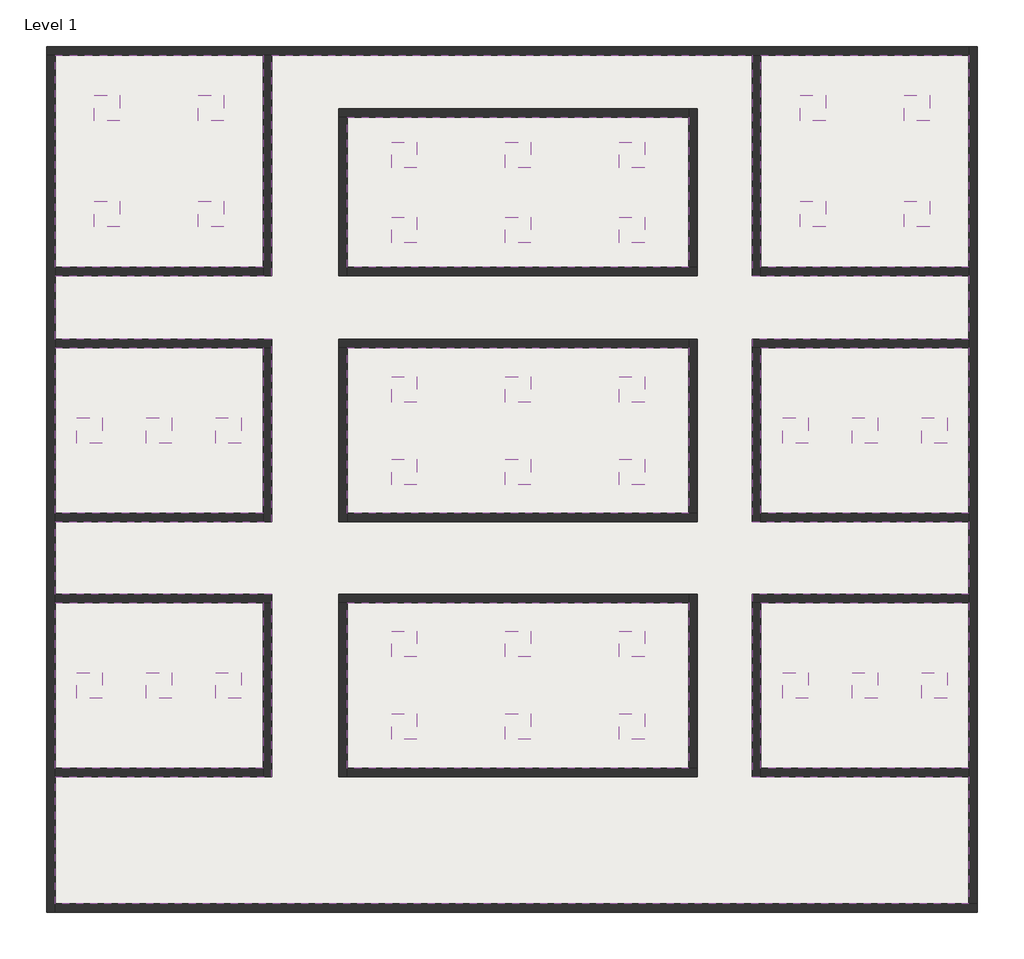
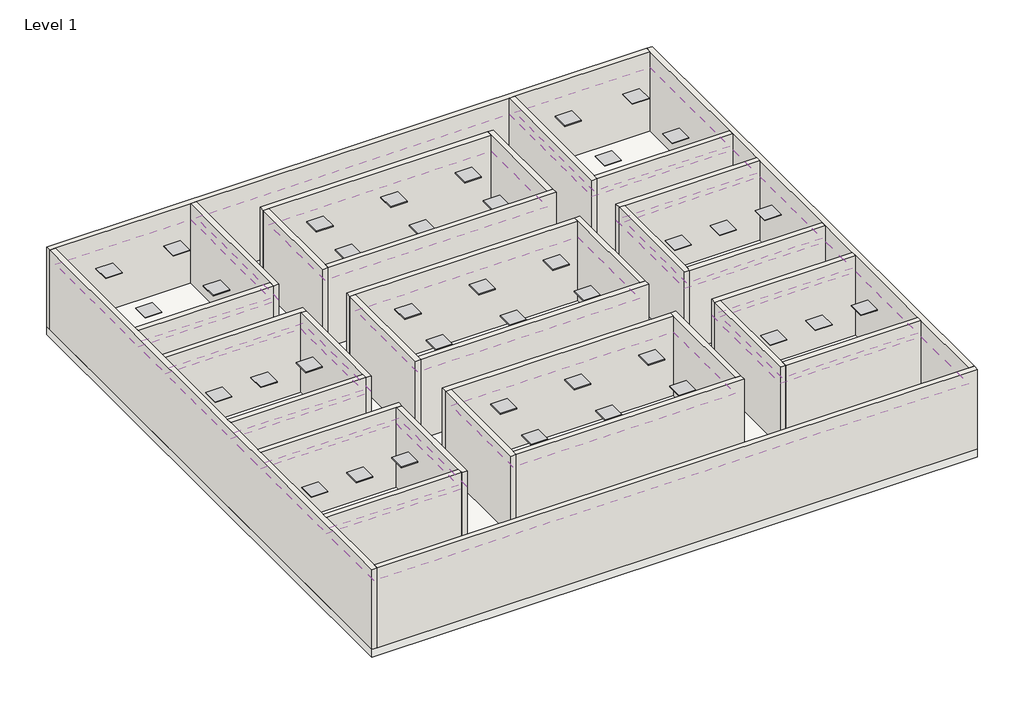
# One storey: 38 light fixtures, 32 walls, 11 coverings, 1 slab.
"""IFC4 building model written with IfcOpenShell, lengths in millimetres."""

import ifcopenshell
import ifcopenshell.guid

model = None  # the IFC model being written
_history = None  # IfcOwnerHistory: only IFC2X3 demands one
_inside = {}  # id of a spatial element -> (the spatial element, [elements in it])
_under = {}  # id of a project, library or spatial element -> (it, [spatial elements below it])
_declared = {}  # id of a project -> (the project, [libraries it declares])
_typed = {}  # id of a type object -> (the type object, [elements of that type])
_made_of = {}  # id of a material, layer set ... -> (it, [elements and type objects made of it])


def new_model(schema):
    """Start an empty IFC model of exactly this schema.

    Asked for "IFC4X3", IfcOpenShell would pick the latest addendum, in which some entities
    have other attributes; the version numbers below select the first issue.
    IFC2X3 requires an IfcOwnerHistory on every rooted entity: one is made here for all.
    """
    global model, _history
    if schema == "IFC4X3":
        model = ifcopenshell.file(schema_version=(4, 3, 0, 0))
    else:
        model = ifcopenshell.file(schema=schema)
    _inside.clear()
    _under.clear()
    _declared.clear()
    _typed.clear()
    _made_of.clear()
    _history = None
    if model.schema == "IFC2X3":
        org = make("IfcOrganization", Name="unknown")
        user = make(
            "IfcPersonAndOrganization",
            ThePerson=make("IfcPerson", FamilyName="unknown"),
            TheOrganization=org,
        )
        app = make(
            "IfcApplication",
            ApplicationDeveloper=org,
            Version="unknown",
            ApplicationFullName="unknown",
            ApplicationIdentifier="unknown",
        )
        _history = make(
            "IfcOwnerHistory",
            OwningUser=user,
            OwningApplication=app,
            ChangeAction="ADDED",
            CreationDate=0,
        )
    return model


def make(cls, **values):
    """One entity of the class cls with the attributes given. An attribute that is None is left unset."""
    return model.create_entity(
        cls, **{name: value for name, value in values.items() if value is not None}
    )


def rooted(cls, **values):
    """An entity with a GlobalId (a new one), such as an element, a storey or a relation."""
    return make(cls, GlobalId=ifcopenshell.guid.new(), OwnerHistory=_history, **values)


def si_unit(unit_type, name, prefix=None):
    """IfcSIUnit, for example si_unit("LENGTHUNIT", "METRE", prefix="MILLI")."""
    return make("IfcSIUnit", UnitType=unit_type, Prefix=prefix, Name=name)


def assignment(units):
    """IfcUnitAssignment: the units of a project."""
    return None if units is None else make("IfcUnitAssignment", Units=units)


def point(xyz):
    """IfcCartesianPoint."""
    return None if xyz is None else make("IfcCartesianPoint", Coordinates=xyz)


def direction(xyz):
    """IfcDirection."""
    return None if xyz is None else make("IfcDirection", DirectionRatios=xyz)


def frame(location, z_axis=None, x_axis=None):
    """IfcAxis2Placement3D, a coordinate frame: its origin and axes. An axis left out is left unset."""
    return make(
        "IfcAxis2Placement3D",
        Location=point(location),
        Axis=direction(z_axis),
        RefDirection=direction(x_axis),
    )


def origin():
    """The frame at (0, 0, 0) with its axes left unset."""
    return frame((0.0, 0.0, 0.0))


def origin_with_axes():
    """The frame at (0, 0, 0) with the z axis (0, 0, 1) and the x axis (1, 0, 0) written out."""
    return frame((0.0, 0.0, 0.0), z_axis=(0.0, 0.0, 1.0), x_axis=(1.0, 0.0, 0.0))


def place(relative_to, where):
    """IfcLocalPlacement: puts the frame where relative to a parent placement (None: the world)."""
    return make(
        "IfcLocalPlacement", PlacementRelTo=relative_to, RelativePlacement=where
    )


def context(
    kind, dimensions, precision=None, world=None, true_north=None, identifier=None
):
    """IfcGeometricRepresentationContext, for example the 3D "Model" context."""
    return make(
        "IfcGeometricRepresentationContext",
        ContextIdentifier=identifier,
        ContextType=kind,
        CoordinateSpaceDimension=dimensions,
        Precision=precision,
        WorldCoordinateSystem=world,
        TrueNorth=true_north,
    )


def project(units=None, contexts=None):
    """IfcProject with its units and contexts."""
    return rooted(
        "IfcProject",
        Name="project",
        RepresentationContexts=contexts,
        UnitsInContext=assignment(units),
    )


def spatial(cls, under=None, at=None, **own):
    """A site, building, storey or space (cls), placed at a placement, below another one or the project."""
    s = rooted(cls, ObjectPlacement=at, **own)
    if under is not None:
        _under.setdefault(under.id(), (under, []))[1].append(s)
    return s


def polyline(points):
    """IfcPolyline through the points."""
    return make("IfcPolyline", Points=[point(p) for p in points])


def outline(outer, holes=None, kind="AREA"):
    """IfcArbitraryClosedProfileDef: a profile drawn as a closed curve; with holes, ...WithVoids."""
    if holes is None:
        return make("IfcArbitraryClosedProfileDef", ProfileType=kind, OuterCurve=outer)
    return make(
        "IfcArbitraryProfileDefWithVoids",
        ProfileType=kind,
        OuterCurve=outer,
        InnerCurves=holes,
    )


def extrude(swept, where, along, depth):
    """IfcExtrudedAreaSolid: the profile swept, set in the frame where, extruded along a direction by depth."""
    return make(
        "IfcExtrudedAreaSolid",
        SweptArea=swept,
        Position=where,
        ExtrudedDirection=direction(along),
        Depth=depth,
    )


def faces_of(points, faces, orient=None, outer=None):
    """IfcFace entities. A face is a list of loops; a loop is a list of indices into points, from 0.

    orient and outer hold one flag for each loop. By default every Orientation is true, the
    first loop of a face is its IfcFaceOuterBound and the others are IfcFaceBound.
    """
    made = []
    for i, loops in enumerate(faces):
        bounds = []
        for j, loop in enumerate(loops):
            is_outer = j == 0 if outer is None else outer[i][j]
            bounds.append(
                make(
                    "IfcFaceOuterBound" if is_outer else "IfcFaceBound",
                    Bound=make("IfcPolyLoop", Polygon=[points[k] for k in loop]),
                    Orientation=True if orient is None else orient[i][j],
                )
            )
        made.append(make("IfcFace", Bounds=bounds))
    return made


def faceted_brep(points, faces, orient=None, outer=None, voids=None):
    """IfcFacetedBrep: a solid bounded by flat faces; with voids (closed shells), ...WithVoids."""
    shared = [point(p) for p in points]
    hull = make("IfcClosedShell", CfsFaces=faces_of(shared, faces, orient, outer))
    if voids is None:
        return make("IfcFacetedBrep", Outer=hull)
    return make(
        "IfcFacetedBrepWithVoids",
        Outer=hull,
        Voids=[
            make(cls, CfsFaces=faces_of(shared, fs, o, b)) for cls, fs, o, b in voids
        ],
    )


def shape(context_of_items, identifier, shape_type, items):
    """IfcShapeRepresentation: the items that make up one representation, for example the "Body"."""
    return make(
        "IfcShapeRepresentation",
        ContextOfItems=context_of_items,
        RepresentationIdentifier=identifier,
        RepresentationType=shape_type,
        Items=items,
    )


def source(mapping_origin, context_of_items, identifier, shape_type, items):
    """IfcRepresentationMap: a shape defined once, which mapped items show again and again."""
    return make(
        "IfcRepresentationMap",
        MappingOrigin=mapping_origin,
        MappedRepresentation=shape(context_of_items, identifier, shape_type, items),
    )


def transform(
    local_origin,
    x_axis=None,
    y_axis=None,
    z_axis=None,
    scale=None,
    scale2=None,
    scale3=None,
    uniform=True,
):
    """IfcCartesianTransformationOperator3D, or its non-uniform kind. x_axis, y_axis, z_axis: its Axis1, 2, 3."""
    if uniform:
        return make(
            "IfcCartesianTransformationOperator3D",
            Axis1=direction(x_axis),
            Axis2=direction(y_axis),
            LocalOrigin=point(local_origin),
            Scale=scale,
            Axis3=direction(z_axis),
        )
    return make(
        "IfcCartesianTransformationOperator3DnonUniform",
        Axis1=direction(x_axis),
        Axis2=direction(y_axis),
        LocalOrigin=point(local_origin),
        Scale=scale,
        Axis3=direction(z_axis),
        Scale2=scale2,
        Scale3=scale3,
    )


def mapped(mapping_source, mapping_target):
    """IfcMappedItem: shows the shape of a source again, moved by a transform."""
    return make(
        "IfcMappedItem", MappingSource=mapping_source, MappingTarget=mapping_target
    )


def made_of(thing, what):
    """Note that an element or type object is made of a material, layer set ...; save() writes the relation."""
    if what is not None:
        _made_of.setdefault(what.id(), (what, []))[1].append(thing)
    return thing


def element(
    cls,
    number,
    at=None,
    inside=None,
    cuts=None,
    type_object=None,
    material=None,
    context=None,
    identifier="Body",
    shape_type=None,
    held_by="IfcProductDefinitionShape",
    body=None,
    shapes=None,
    **own,
):
    """One element of the class cls, such as IfcWall. Its Tag is "e" and its number.

    at: its placement. inside: the storey or other place that contains it. cuts: it is an
    opening in that element (IfcRelVoidsElement). A single representation is given by context,
    identifier, shape_type and body (its items); several are given by shapes. held_by: the class
    of the entity that holds the representations. save() writes the other relations.
    """
    e = rooted(cls, Tag="e%d" % number, ObjectPlacement=at, **own)
    if body is not None:
        shapes = [shape(context, identifier, shape_type, body)]
    if shapes is not None:
        e.Representation = make(held_by, Representations=shapes)
    if inside is not None:
        _inside.setdefault(inside.id(), (inside, []))[1].append(e)
    if cuts is not None:
        rooted(
            "IfcRelVoidsElement", RelatingBuildingElement=cuts, RelatedOpeningElement=e
        )
    if type_object is not None:
        _typed.setdefault(type_object.id(), (type_object, []))[1].append(e)
    return made_of(e, material)


def aggregate(whole, parts):
    """IfcRelAggregates: a whole, such as a stair, and the parts it consists of."""
    return rooted("IfcRelAggregates", RelatingObject=whole, RelatedObjects=parts)


def save(model, path):
    """Write the relations noted so far, then the file.

    IfcRelAggregates (storeys below a building ...), IfcRelContainedInSpatialStructure (elements
    in a storey), IfcRelDefinesByType, IfcRelAssociatesMaterial and IfcRelDeclares: one each for
    every whole, place, type object, material and project.
    """
    for whole, parts in _under.values():
        aggregate(whole, parts)
    for where, things in _inside.values():
        rooted(
            "IfcRelContainedInSpatialStructure",
            RelatedElements=things,
            RelatingStructure=where,
        )
    for kind, things in _typed.values():
        rooted("IfcRelDefinesByType", RelatedObjects=things, RelatingType=kind)
    for what, things in _made_of.values():
        rooted("IfcRelAssociatesMaterial", RelatedObjects=things, RelatingMaterial=what)
    for by, libraries in _declared.values():
        rooted("IfcRelDeclares", RelatingContext=by, RelatedDefinitions=libraries)
    model.write(path)


def simple_lights_a_61f39cf9(model_context):
    return source(origin(), model_context, "Body", "SweptSolid", [
        extrude(outline(polyline([(300.0, 300.0), (300.0, -300.0), (-300.0, -300.0), (-300.0, 300.0), (300.0, 300.0)])), frame((0.0, 0.0, -30.0), z_axis=(0.0, 0.0, 1.0), x_axis=(1.0, 0.0, 0.0)), (0.0, 0.0, 1.0), 30.0),
    ])


model = new_model("IFC4")

# Units and contexts
model_context = context("Model", 3, world=origin())
ifc_project = project(units=[si_unit("LENGTHUNIT", "METRE", prefix="MILLI")], contexts=[model_context])

# Site, building, storey
site = spatial("IfcSite", under=ifc_project)
building = spatial("IfcBuilding", under=site)
storey = spatial("IfcBuildingStorey", under=building, Name="Level 1", Elevation=0.0)

# Coverings
placement = place(None, origin())
element("IfcCovering", 1, ObjectType="2' x 4' ACT System", at=placement, inside=storey, context=model_context, shape_type="SweptSolid", body=[
    extrude(outline(polyline([(-11709.662063, 12460.3552234), (-6809.662063, 12460.3552234), (-6809.662063, 7460.3552234), (-11709.662063, 7460.3552234), (-11709.662063, 12460.3552234)])), frame((0.0, 0.0, 2438.4), z_axis=(0.0, 0.0, 1.0), x_axis=(1.0, 0.0, 0.0)), (0.0, 0.0, 1.0), 57.15),
])
element("IfcCovering", 2, ObjectType="2' x 4' ACT System", at=placement, inside=storey, context=model_context, shape_type="SweptSolid", body=[
    extrude(outline(polyline([(-6609.662063, 7260.3552234), (-6609.662063, 12460.3552234), (4722.664183, 12460.3552234), (4722.664183, 7260.3552234), (9822.664183, 7260.3552234), (9822.664183, 5760.3552234), (4722.664183, 5760.3552234), (4722.664183, 1460.3552234), (9822.664183, 1460.3552234), (9822.664183, -239.6447766), (4722.664183, -239.6447766), (4722.664183, -4539.6447766), (9822.664183, -4539.6447766), (9822.664183, -7539.6447766), (-11709.662063, -7539.6447766), (-11709.662063, -4539.6447766), (-6609.662063, -4539.6447766), (-6609.662063, -239.6447766), (-11709.662063, -239.6447766), (-11709.662063, 1460.3552234), (-6609.662063, 1460.3552234), (-6609.662063, 5760.3552234), (-11709.662063, 5760.3552234), (-11709.662063, 7260.3552234), (-6609.662063, 7260.3552234)]), holes=[polyline([(3422.664183, 7260.3552234), (3422.664183, 11191.3898121), (-5023.4293583, 11191.3898121), (-5023.4293583, 7260.3552234), (3422.664183, 7260.3552234)]), polyline([(3422.664183, 1460.3552234), (3422.664183, 5760.3552234), (-5023.4293583, 5760.3552234), (-5023.4293583, 1460.3552234), (3422.664183, 1460.3552234)]), polyline([(3422.664183, -4539.6447766), (3422.664183, -239.6447766), (-5023.4293583, -239.6447766), (-5023.4293583, -4539.6447766), (3422.664183, -4539.6447766)])]), frame((0.0, 0.0, 2438.4), z_axis=(0.0, 0.0, 1.0), x_axis=(1.0, 0.0, 0.0)), (0.0, 0.0, 1.0), 57.15),
])
element("IfcCovering", 3, ObjectType="2' x 4' ACT System", at=placement, inside=storey, context=model_context, shape_type="SweptSolid", body=[
    extrude(outline(polyline([(-4823.4293583, 10991.3898121), (3222.664183, 10991.3898121), (3222.664183, 7460.3552234), (-4823.4293583, 7460.3552234), (-4823.4293583, 10991.3898121)])), frame((0.0, 0.0, 2438.4), z_axis=(0.0, 0.0, 1.0), x_axis=(1.0, 0.0, 0.0)), (0.0, 0.0, 1.0), 57.15),
])
element("IfcCovering", 4, ObjectType="2' x 4' ACT System", at=placement, inside=storey, context=model_context, shape_type="SweptSolid", body=[
    extrude(outline(polyline([(4922.664183, 7460.3552234), (4922.664183, 12460.3552234), (9822.664183, 12460.3552234), (9822.664183, 7460.3552234), (4922.664183, 7460.3552234)])), frame((0.0, 0.0, 2438.4), z_axis=(0.0, 0.0, 1.0), x_axis=(1.0, 0.0, 0.0)), (0.0, 0.0, 1.0), 57.15),
])
element("IfcCovering", 5, ObjectType="2' x 4' ACT System", at=placement, inside=storey, context=model_context, shape_type="SweptSolid", body=[
    extrude(outline(polyline([(4922.664183, 5560.3552234), (9822.664183, 5560.3552234), (9822.664183, 1660.3552234), (4922.664183, 1660.3552234), (4922.664183, 5560.3552234)])), frame((0.0, 0.0, 2438.4), z_axis=(0.0, 0.0, 1.0), x_axis=(1.0, 0.0, 0.0)), (0.0, 0.0, 1.0), 57.15),
])
element("IfcCovering", 6, ObjectType="2' x 4' ACT System", at=placement, inside=storey, context=model_context, shape_type="SweptSolid", body=[
    extrude(outline(polyline([(4922.664183, -439.6447766), (9822.664183, -439.6447766), (9822.664183, -4339.6447766), (4922.664183, -4339.6447766), (4922.664183, -439.6447766)])), frame((0.0, 0.0, 2438.4), z_axis=(0.0, 0.0, 1.0), x_axis=(1.0, 0.0, 0.0)), (0.0, 0.0, 1.0), 57.15),
])
element("IfcCovering", 7, ObjectType="2' x 4' ACT System", at=placement, inside=storey, context=model_context, shape_type="SweptSolid", body=[
    extrude(outline(polyline([(-4823.4293583, -439.6447766), (3222.664183, -439.6447766), (3222.664183, -4339.6447766), (-4823.4293583, -4339.6447766), (-4823.4293583, -439.6447766)])), frame((0.0, 0.0, 2438.4), z_axis=(0.0, 0.0, 1.0), x_axis=(1.0, 0.0, 0.0)), (0.0, 0.0, 1.0), 57.15),
])
element("IfcCovering", 8, ObjectType="2' x 4' ACT System", at=placement, inside=storey, context=model_context, shape_type="SweptSolid", body=[
    extrude(outline(polyline([(-11709.662063, -4339.6447766), (-11709.662063, -439.6447766), (-6809.662063, -439.6447766), (-6809.662063, -4339.6447766), (-11709.662063, -4339.6447766)])), frame((0.0, 0.0, 2438.4), z_axis=(0.0, 0.0, 1.0), x_axis=(1.0, 0.0, 0.0)), (0.0, 0.0, 1.0), 57.15),
])
element("IfcCovering", 9, ObjectType="2' x 4' ACT System", at=placement, inside=storey, context=model_context, shape_type="SweptSolid", body=[
    extrude(outline(polyline([(-11709.662063, 1660.3552234), (-11709.662063, 5560.3552234), (-6809.662063, 5560.3552234), (-6809.662063, 1660.3552234), (-11709.662063, 1660.3552234)])), frame((0.0, 0.0, 2438.4), z_axis=(0.0, 0.0, 1.0), x_axis=(1.0, 0.0, 0.0)), (0.0, 0.0, 1.0), 57.15),
])
element("IfcCovering", 10, ObjectType="2' x 4' ACT System", at=placement, inside=storey, context=model_context, shape_type="SweptSolid", body=[
    extrude(outline(polyline([(-4823.4293583, 5560.3552234), (3222.664183, 5560.3552234), (3222.664183, 1660.3552234), (-4823.4293583, 1660.3552234), (-4823.4293583, 5560.3552234)])), frame((0.0, 0.0, 2438.4), z_axis=(0.0, 0.0, 1.0), x_axis=(1.0, 0.0, 0.0)), (0.0, 0.0, 1.0), 57.15),
])
element("IfcCovering", 11, ObjectType="2' x 4' ACT System", at=placement, inside=storey, context=model_context, shape_type="SweptSolid", body=[
    extrude(outline(polyline([(4922.664183, 5560.3552234), (9822.664183, 5560.3552234), (9822.664183, 1660.3552234), (4922.664183, 1660.3552234), (4922.664183, 5560.3552234)])), frame((0.0, 0.0, 2438.4), z_axis=(0.0, 0.0, 1.0), x_axis=(1.0, 0.0, 0.0)), (0.0, 0.0, 1.0), 57.15),
])

# Light fixtures
simple_lights_a_shape = simple_lights_a_61f39cf9(model_context)
element("IfcLightFixture", 12, ObjectType="Simple Lights : A", at=placement, inside=storey, context=model_context, shape_type="MappedRepresentation", body=[
    mapped(simple_lights_a_shape, transform((-10892.9953964, -2389.6447766, 2531.4000022), x_axis=(1.0, 0.0, 0.0), y_axis=(0.0, 1.0, 0.0), z_axis=(0.0, 0.0, 1.0))),
])
element("IfcLightFixture", 13, ObjectType="Simple Lights : A", at=placement, inside=storey, context=model_context, shape_type="MappedRepresentation", body=[
    mapped(simple_lights_a_shape, transform((-9259.662063, -2389.6447766, 2531.4000022), x_axis=(1.0, 0.0, 0.0), y_axis=(0.0, 1.0, 0.0), z_axis=(0.0, 0.0, 1.0))),
])
element("IfcLightFixture", 14, ObjectType="Simple Lights : A", at=placement, inside=storey, context=model_context, shape_type="MappedRepresentation", body=[
    mapped(simple_lights_a_shape, transform((-7626.3287297, -2389.6447766, 2531.4000022), x_axis=(1.0, 0.0, 0.0), y_axis=(0.0, 1.0, 0.0), z_axis=(0.0, 0.0, 1.0))),
])
element("IfcLightFixture", 15, ObjectType="Simple Lights : A", at=placement, inside=storey, context=model_context, shape_type="MappedRepresentation", body=[
    mapped(simple_lights_a_shape, transform((-3482.4137681, -3364.6447766, 2531.4000022), x_axis=(1.0, 0.0, 0.0), y_axis=(0.0, 1.0, 0.0), z_axis=(0.0, 0.0, 1.0))),
])
element("IfcLightFixture", 16, ObjectType="Simple Lights : A", at=placement, inside=storey, context=model_context, shape_type="MappedRepresentation", body=[
    mapped(simple_lights_a_shape, transform((-800.3825877, -3364.6447766, 2531.4000022), x_axis=(1.0, 0.0, 0.0), y_axis=(0.0, 1.0, 0.0), z_axis=(0.0, 0.0, 1.0))),
])
element("IfcLightFixture", 17, ObjectType="Simple Lights : A", at=placement, inside=storey, context=model_context, shape_type="MappedRepresentation", body=[
    mapped(simple_lights_a_shape, transform((1881.6485928, -3364.6447766, 2531.4000022), x_axis=(1.0, 0.0, 0.0), y_axis=(0.0, 1.0, 0.0), z_axis=(0.0, 0.0, 1.0))),
])
element("IfcLightFixture", 18, ObjectType="Simple Lights : A", at=placement, inside=storey, context=model_context, shape_type="MappedRepresentation", body=[
    mapped(simple_lights_a_shape, transform((-3482.4137681, -1414.6447766, 2531.4000022), x_axis=(1.0, 0.0, 0.0), y_axis=(0.0, 1.0, 0.0), z_axis=(0.0, 0.0, 1.0))),
])
element("IfcLightFixture", 19, ObjectType="Simple Lights : A", at=placement, inside=storey, context=model_context, shape_type="MappedRepresentation", body=[
    mapped(simple_lights_a_shape, transform((-800.3825877, -1414.6447766, 2531.4000022), x_axis=(1.0, 0.0, 0.0), y_axis=(0.0, 1.0, 0.0), z_axis=(0.0, 0.0, 1.0))),
])
element("IfcLightFixture", 20, ObjectType="Simple Lights : A", at=placement, inside=storey, context=model_context, shape_type="MappedRepresentation", body=[
    mapped(simple_lights_a_shape, transform((1881.6485928, -1414.6447766, 2531.4000022), x_axis=(1.0, 0.0, 0.0), y_axis=(0.0, 1.0, 0.0), z_axis=(0.0, 0.0, 1.0))),
])
element("IfcLightFixture", 21, ObjectType="Simple Lights : A", at=placement, inside=storey, context=model_context, shape_type="MappedRepresentation", body=[
    mapped(simple_lights_a_shape, transform((5739.3308497, -2389.6447766, 2531.4000022), x_axis=(1.0, 0.0, 0.0), y_axis=(0.0, 1.0, 0.0), z_axis=(0.0, 0.0, 1.0))),
])
element("IfcLightFixture", 22, ObjectType="Simple Lights : A", at=placement, inside=storey, context=model_context, shape_type="MappedRepresentation", body=[
    mapped(simple_lights_a_shape, transform((7372.664183, -2389.6447766, 2531.4000022), x_axis=(1.0, 0.0, 0.0), y_axis=(0.0, 1.0, 0.0), z_axis=(0.0, 0.0, 1.0))),
])
element("IfcLightFixture", 23, ObjectType="Simple Lights : A", at=placement, inside=storey, context=model_context, shape_type="MappedRepresentation", body=[
    mapped(simple_lights_a_shape, transform((9005.9975163, -2389.6447766, 2531.4000022), x_axis=(1.0, 0.0, 0.0), y_axis=(0.0, 1.0, 0.0), z_axis=(0.0, 0.0, 1.0))),
])
element("IfcLightFixture", 24, ObjectType="Simple Lights : A", at=placement, inside=storey, context=model_context, shape_type="MappedRepresentation", body=[
    mapped(simple_lights_a_shape, transform((5739.3308497, 3610.3552234, 2531.4000022), x_axis=(1.0, 0.0, 0.0), y_axis=(0.0, 1.0, 0.0), z_axis=(0.0, 0.0, 1.0))),
])
element("IfcLightFixture", 25, ObjectType="Simple Lights : A", at=placement, inside=storey, context=model_context, shape_type="MappedRepresentation", body=[
    mapped(simple_lights_a_shape, transform((7372.664183, 3610.3552234, 2531.4000022), x_axis=(1.0, 0.0, 0.0), y_axis=(0.0, 1.0, 0.0), z_axis=(0.0, 0.0, 1.0))),
])
element("IfcLightFixture", 26, ObjectType="Simple Lights : A", at=placement, inside=storey, context=model_context, shape_type="MappedRepresentation", body=[
    mapped(simple_lights_a_shape, transform((9005.9975163, 3610.3552234, 2531.4000022), x_axis=(1.0, 0.0, 0.0), y_axis=(0.0, 1.0, 0.0), z_axis=(0.0, 0.0, 1.0))),
])
element("IfcLightFixture", 27, ObjectType="Simple Lights : A", at=placement, inside=storey, context=model_context, shape_type="MappedRepresentation", body=[
    mapped(simple_lights_a_shape, transform((-3482.4137681, 2635.3552234, 2531.4000022), x_axis=(1.0, 0.0, 0.0), y_axis=(0.0, 1.0, 0.0), z_axis=(0.0, 0.0, 1.0))),
])
element("IfcLightFixture", 28, ObjectType="Simple Lights : A", at=placement, inside=storey, context=model_context, shape_type="MappedRepresentation", body=[
    mapped(simple_lights_a_shape, transform((-800.3825877, 2635.3552234, 2531.4000022), x_axis=(1.0, 0.0, 0.0), y_axis=(0.0, 1.0, 0.0), z_axis=(0.0, 0.0, 1.0))),
])
element("IfcLightFixture", 29, ObjectType="Simple Lights : A", at=placement, inside=storey, context=model_context, shape_type="MappedRepresentation", body=[
    mapped(simple_lights_a_shape, transform((1881.6485928, 2635.3552234, 2531.4000022), x_axis=(1.0, 0.0, 0.0), y_axis=(0.0, 1.0, 0.0), z_axis=(0.0, 0.0, 1.0))),
])
element("IfcLightFixture", 30, ObjectType="Simple Lights : A", at=placement, inside=storey, context=model_context, shape_type="MappedRepresentation", body=[
    mapped(simple_lights_a_shape, transform((-3482.4137681, 4585.3552234, 2531.4000022), x_axis=(1.0, 0.0, 0.0), y_axis=(0.0, 1.0, 0.0), z_axis=(0.0, 0.0, 1.0))),
])
element("IfcLightFixture", 31, ObjectType="Simple Lights : A", at=placement, inside=storey, context=model_context, shape_type="MappedRepresentation", body=[
    mapped(simple_lights_a_shape, transform((-800.3825877, 4585.3552234, 2531.4000022), x_axis=(1.0, 0.0, 0.0), y_axis=(0.0, 1.0, 0.0), z_axis=(0.0, 0.0, 1.0))),
])
element("IfcLightFixture", 32, ObjectType="Simple Lights : A", at=placement, inside=storey, context=model_context, shape_type="MappedRepresentation", body=[
    mapped(simple_lights_a_shape, transform((1881.6485928, 4585.3552234, 2531.4000022), x_axis=(1.0, 0.0, 0.0), y_axis=(0.0, 1.0, 0.0), z_axis=(0.0, 0.0, 1.0))),
])
element("IfcLightFixture", 33, ObjectType="Simple Lights : A", at=placement, inside=storey, context=model_context, shape_type="MappedRepresentation", body=[
    mapped(simple_lights_a_shape, transform((-10892.9953964, 3610.3552234, 2531.4000022), x_axis=(1.0, 0.0, 0.0), y_axis=(0.0, 1.0, 0.0), z_axis=(0.0, 0.0, 1.0))),
])
element("IfcLightFixture", 34, ObjectType="Simple Lights : A", at=placement, inside=storey, context=model_context, shape_type="MappedRepresentation", body=[
    mapped(simple_lights_a_shape, transform((-9259.662063, 3610.3552234, 2531.4000022), x_axis=(1.0, 0.0, 0.0), y_axis=(0.0, 1.0, 0.0), z_axis=(0.0, 0.0, 1.0))),
])
element("IfcLightFixture", 35, ObjectType="Simple Lights : A", at=placement, inside=storey, context=model_context, shape_type="MappedRepresentation", body=[
    mapped(simple_lights_a_shape, transform((-7626.3287297, 3610.3552234, 2531.4000022), x_axis=(1.0, 0.0, 0.0), y_axis=(0.0, 1.0, 0.0), z_axis=(0.0, 0.0, 1.0))),
])
element("IfcLightFixture", 36, ObjectType="Simple Lights : A", at=placement, inside=storey, context=model_context, shape_type="MappedRepresentation", body=[
    mapped(simple_lights_a_shape, transform((-10484.662063, 8710.3552234, 2531.4000022), x_axis=(1.0, 0.0, 0.0), y_axis=(0.0, 1.0, 0.0), z_axis=(0.0, 0.0, 1.0))),
])
element("IfcLightFixture", 37, ObjectType="Simple Lights : A", at=placement, inside=storey, context=model_context, shape_type="MappedRepresentation", body=[
    mapped(simple_lights_a_shape, transform((-8034.662063, 8710.3552234, 2531.4000022), x_axis=(1.0, 0.0, 0.0), y_axis=(0.0, 1.0, 0.0), z_axis=(0.0, 0.0, 1.0))),
])
element("IfcLightFixture", 38, ObjectType="Simple Lights : A", at=placement, inside=storey, context=model_context, shape_type="MappedRepresentation", body=[
    mapped(simple_lights_a_shape, transform((-10484.662063, 11210.3552234, 2531.4000022), x_axis=(1.0, 0.0, 0.0), y_axis=(0.0, 1.0, 0.0), z_axis=(0.0, 0.0, 1.0))),
])
element("IfcLightFixture", 39, ObjectType="Simple Lights : A", at=placement, inside=storey, context=model_context, shape_type="MappedRepresentation", body=[
    mapped(simple_lights_a_shape, transform((-8034.662063, 11210.3552234, 2531.4000022), x_axis=(1.0, 0.0, 0.0), y_axis=(0.0, 1.0, 0.0), z_axis=(0.0, 0.0, 1.0))),
])
element("IfcLightFixture", 40, ObjectType="Simple Lights : A", at=placement, inside=storey, context=model_context, shape_type="MappedRepresentation", body=[
    mapped(simple_lights_a_shape, transform((-3482.4137681, 8343.1138706, 2531.4000022), x_axis=(1.0, 0.0, 0.0), y_axis=(0.0, 1.0, 0.0), z_axis=(0.0, 0.0, 1.0))),
])
element("IfcLightFixture", 41, ObjectType="Simple Lights : A", at=placement, inside=storey, context=model_context, shape_type="MappedRepresentation", body=[
    mapped(simple_lights_a_shape, transform((-800.3825877, 8343.1138706, 2531.4000022), x_axis=(1.0, 0.0, 0.0), y_axis=(0.0, 1.0, 0.0), z_axis=(0.0, 0.0, 1.0))),
])
element("IfcLightFixture", 42, ObjectType="Simple Lights : A", at=placement, inside=storey, context=model_context, shape_type="MappedRepresentation", body=[
    mapped(simple_lights_a_shape, transform((1881.6485928, 8343.1138706, 2531.4000022), x_axis=(1.0, 0.0, 0.0), y_axis=(0.0, 1.0, 0.0), z_axis=(0.0, 0.0, 1.0))),
])
element("IfcLightFixture", 43, ObjectType="Simple Lights : A", at=placement, inside=storey, context=model_context, shape_type="MappedRepresentation", body=[
    mapped(simple_lights_a_shape, transform((-3482.4137681, 10108.6311649, 2531.4000022), x_axis=(1.0, 0.0, 0.0), y_axis=(0.0, 1.0, 0.0), z_axis=(0.0, 0.0, 1.0))),
])
element("IfcLightFixture", 44, ObjectType="Simple Lights : A", at=placement, inside=storey, context=model_context, shape_type="MappedRepresentation", body=[
    mapped(simple_lights_a_shape, transform((-800.3825877, 10108.6311649, 2531.4000022), x_axis=(1.0, 0.0, 0.0), y_axis=(0.0, 1.0, 0.0), z_axis=(0.0, 0.0, 1.0))),
])
element("IfcLightFixture", 45, ObjectType="Simple Lights : A", at=placement, inside=storey, context=model_context, shape_type="MappedRepresentation", body=[
    mapped(simple_lights_a_shape, transform((1881.6485928, 10108.6311649, 2531.4000022), x_axis=(1.0, 0.0, 0.0), y_axis=(0.0, 1.0, 0.0), z_axis=(0.0, 0.0, 1.0))),
])
element("IfcLightFixture", 46, ObjectType="Simple Lights : A", at=placement, inside=storey, context=model_context, shape_type="MappedRepresentation", body=[
    mapped(simple_lights_a_shape, transform((6147.664183, 8710.3552234, 2531.4000022), x_axis=(1.0, 0.0, 0.0), y_axis=(0.0, 1.0, 0.0), z_axis=(0.0, 0.0, 1.0))),
])
element("IfcLightFixture", 47, ObjectType="Simple Lights : A", at=placement, inside=storey, context=model_context, shape_type="MappedRepresentation", body=[
    mapped(simple_lights_a_shape, transform((8597.664183, 8710.3552234, 2531.4000022), x_axis=(1.0, 0.0, 0.0), y_axis=(0.0, 1.0, 0.0), z_axis=(0.0, 0.0, 1.0))),
])
element("IfcLightFixture", 48, ObjectType="Simple Lights : A", at=placement, inside=storey, context=model_context, shape_type="MappedRepresentation", body=[
    mapped(simple_lights_a_shape, transform((6147.664183, 11210.3552234, 2531.4000022), x_axis=(1.0, 0.0, 0.0), y_axis=(0.0, 1.0, 0.0), z_axis=(0.0, 0.0, 1.0))),
])
element("IfcLightFixture", 49, ObjectType="Simple Lights : A", at=placement, inside=storey, context=model_context, shape_type="MappedRepresentation", body=[
    mapped(simple_lights_a_shape, transform((8597.664183, 11210.3552234, 2531.4000022), x_axis=(1.0, 0.0, 0.0), y_axis=(0.0, 1.0, 0.0), z_axis=(0.0, 0.0, 1.0))),
])

# Slab
element("IfcSlab", 50, ObjectType="Generic - 12\"", at=placement, inside=storey, context=model_context, shape_type="SweptSolid", body=[
    extrude(outline(polyline([(10022.664183, 12660.3552234), (10022.664183, -7739.6447766), (-11909.662063, -7739.6447766), (-11909.662063, 12660.3552234), (10022.664183, 12660.3552234)])), frame((0.0, 0.0, -304.8), z_axis=(0.0, 0.0, 1.0), x_axis=(1.0, 0.0, 0.0)), (0.0, 0.0, 1.0), 304.8),
])

# Walls
element("IfcWall", 51, ObjectType="Generic - 200mm", at=placement, inside=storey, context=model_context, shape_type="Brep", body=[
    faceted_brep([(-11909.662063, 12460.3552234, 0.0), (-11709.662063, 12460.3552234, 0.0), (-6809.662063, 12460.3552234, 0.0), (-6609.662063, 12460.3552234, 0.0), (4722.664183, 12460.3552234, 0.0), (4922.664183, 12460.3552234, 0.0), (9822.664183, 12460.3552234, 0.0), (9822.664183, 12460.3552234, 3048.0), (4922.664183, 12460.3552234, 3048.0), (4722.664183, 12460.3552234, 3048.0), (-6609.662063, 12460.3552234, 3048.0), (-6809.662063, 12460.3552234, 3048.0), (-11709.662063, 12460.3552234, 3048.0), (-11909.662063, 12460.3552234, 3048.0), (-11909.662063, 12660.3552234, 0.0), (-11909.662063, 12660.3552234, 3048.0), (9822.664183, 12660.3552234, 3048.0), (9822.664183, 12660.3552234, 0.0)], [[[0, 1, 2, 3, 4, 5, 6, 7, 8, 9, 10, 11, 12, 13]], [[14, 15, 16, 17]], [[6, 5, 4, 3, 2, 1, 0, 14, 17]], [[0, 13, 15, 14]], [[7, 6, 17, 16]], [[13, 12, 11, 10, 9, 8, 7, 16, 15]]]),
])
element("IfcWall", 52, ObjectType="Generic - 200mm", at=placement, inside=storey, context=model_context, shape_type="Brep", body=[
    faceted_brep([(-11709.662063, -7739.6447766, 0.0), (-11709.662063, -7539.6447766, 0.0), (-11709.662063, -4539.6447766, 0.0), (-11709.662063, -4339.6447766, 0.0), (-11709.662063, -439.6447766, 0.0), (-11709.662063, -239.6447766, 0.0), (-11709.662063, 1460.3552234, 0.0), (-11709.662063, 1660.3552234, 0.0), (-11709.662063, 5560.3552234, 0.0), (-11709.662063, 5760.3552234, 0.0), (-11709.662063, 7260.3552234, 0.0), (-11709.662063, 7460.3552234, 0.0), (-11709.662063, 12460.3552234, 0.0), (-11709.662063, 12460.3552234, 3048.0), (-11709.662063, 7460.3552234, 3048.0), (-11709.662063, 7260.3552234, 3048.0), (-11709.662063, 5760.3552234, 3048.0), (-11709.662063, 5560.3552234, 3048.0), (-11709.662063, 1660.3552234, 3048.0), (-11709.662063, 1460.3552234, 3048.0), (-11709.662063, -239.6447766, 3048.0), (-11709.662063, -439.6447766, 3048.0), (-11709.662063, -4339.6447766, 3048.0), (-11709.662063, -4539.6447766, 3048.0), (-11709.662063, -7539.6447766, 3048.0), (-11709.662063, -7739.6447766, 3048.0), (-11909.662063, -7739.6447766, 0.0), (-11909.662063, -7739.6447766, 3048.0), (-11909.662063, 12460.3552234, 3048.0), (-11909.662063, 12460.3552234, 0.0)], [[[0, 1, 2, 3, 4, 5, 6, 7, 8, 9, 10, 11, 12, 13, 14, 15, 16, 17, 18, 19, 20, 21, 22, 23, 24, 25]], [[26, 27, 28, 29]], [[12, 11, 10, 9, 8, 7, 6, 5, 4, 3, 2, 1, 0, 26, 29]], [[0, 25, 27, 26]], [[13, 12, 29, 28]], [[25, 24, 23, 22, 21, 20, 19, 18, 17, 16, 15, 14, 13, 28, 27]]]),
])
element("IfcWall", 53, ObjectType="Generic - 200mm", at=placement, inside=storey, context=model_context, shape_type="Brep", body=[
    faceted_brep([(10022.664183, -7539.6447766, 0.0), (9822.664183, -7539.6447766, 0.0), (-11709.662063, -7539.6447766, 0.0), (-11709.662063, -7539.6447766, 3048.0), (9822.664183, -7539.6447766, 3048.0), (10022.664183, -7539.6447766, 3048.0), (10022.664183, -7739.6447766, 0.0), (10022.664183, -7739.6447766, 3048.0), (-11709.662063, -7739.6447766, 3048.0), (-11709.662063, -7739.6447766, 0.0)], [[[0, 1, 2, 3, 4, 5]], [[6, 7, 8, 9]], [[2, 1, 0, 6, 9]], [[0, 5, 7, 6]], [[3, 2, 9, 8]], [[5, 4, 3, 8, 7]]]),
])
element("IfcWall", 54, ObjectType="Generic - 200mm", at=placement, inside=storey, context=model_context, shape_type="Brep", body=[
    faceted_brep([(9822.664183, 12660.3552234, 0.0), (9822.664183, 12460.3552234, 0.0), (9822.664183, 7460.3552234, 0.0), (9822.664183, 7260.3552234, 0.0), (9822.664183, 5760.3552234, 0.0), (9822.664183, 5560.3552234, 0.0), (9822.664183, 1660.3552234, 0.0), (9822.664183, 1460.3552234, 0.0), (9822.664183, -239.6447766, 0.0), (9822.664183, -439.6447766, 0.0), (9822.664183, -4339.6447766, 0.0), (9822.664183, -4539.6447766, 0.0), (9822.664183, -7539.6447766, 0.0), (9822.664183, -7539.6447766, 3048.0), (9822.664183, -4539.6447766, 3048.0), (9822.664183, -4339.6447766, 3048.0), (9822.664183, -439.6447766, 3048.0), (9822.664183, -239.6447766, 3048.0), (9822.664183, 1460.3552234, 3048.0), (9822.664183, 1660.3552234, 3048.0), (9822.664183, 5560.3552234, 3048.0), (9822.664183, 5760.3552234, 3048.0), (9822.664183, 7260.3552234, 3048.0), (9822.664183, 7460.3552234, 3048.0), (9822.664183, 12460.3552234, 3048.0), (9822.664183, 12660.3552234, 3048.0), (10022.664183, 12660.3552234, 0.0), (10022.664183, 12660.3552234, 3048.0), (10022.664183, -7539.6447766, 3048.0), (10022.664183, -7539.6447766, 0.0)], [[[0, 1, 2, 3, 4, 5, 6, 7, 8, 9, 10, 11, 12, 13, 14, 15, 16, 17, 18, 19, 20, 21, 22, 23, 24, 25]], [[26, 27, 28, 29]], [[12, 11, 10, 9, 8, 7, 6, 5, 4, 3, 2, 1, 0, 26, 29]], [[0, 25, 27, 26]], [[13, 12, 29, 28]], [[25, 24, 23, 22, 21, 20, 19, 18, 17, 16, 15, 14, 13, 28, 27]]]),
])
element("IfcWall", 55, ObjectType="Generic - 200mm", at=placement, inside=storey, context=model_context, shape_type="Brep", body=[
    faceted_brep([(-6809.662063, -439.6447766, 0.0), (-6809.662063, -4339.6447766, 0.0), (-6809.662063, -4539.6447766, 0.0), (-6809.662063, -4539.6447766, 3048.0), (-6809.662063, -4339.6447766, 3048.0), (-6809.662063, -439.6447766, 3048.0), (-6609.662063, -439.6447766, 0.0), (-6609.662063, -439.6447766, 3048.0), (-6609.662063, -4539.6447766, 3048.0), (-6609.662063, -4539.6447766, 0.0)], [[[0, 1, 2, 3, 4, 5]], [[6, 7, 8, 9]], [[2, 1, 0, 6, 9]], [[3, 2, 9, 8]], [[0, 5, 7, 6]], [[5, 4, 3, 8, 7]]]),
])
element("IfcWall", 56, ObjectType="Generic - 200mm", at=placement, inside=storey, context=model_context, shape_type="SweptSolid", body=[
    extrude(outline(polyline([(-11709.662063, -4339.6447766), (-6809.662063, -4339.6447766), (-6809.662063, -4539.6447766), (-11709.662063, -4539.6447766), (-11709.662063, -4339.6447766)])), origin_with_axes(), (0.0, 0.0, 1.0), 3048.0),
])
element("IfcWall", 57, ObjectType="Generic - 200mm", at=placement, inside=storey, context=model_context, shape_type="Brep", body=[
    faceted_brep([(-11709.662063, -439.6447766, 0.0), (-6809.662063, -439.6447766, 0.0), (-6609.662063, -439.6447766, 0.0), (-6609.662063, -439.6447766, 3048.0), (-6809.662063, -439.6447766, 3048.0), (-11709.662063, -439.6447766, 3048.0), (-11709.662063, -239.6447766, 0.0), (-11709.662063, -239.6447766, 3048.0), (-6609.662063, -239.6447766, 3048.0), (-6609.662063, -239.6447766, 0.0)], [[[0, 1, 2, 3, 4, 5]], [[6, 7, 8, 9]], [[2, 1, 0, 6, 9]], [[0, 5, 7, 6]], [[3, 2, 9, 8]], [[5, 4, 3, 8, 7]]]),
])
element("IfcWall", 58, ObjectType="Generic - 200mm", at=placement, inside=storey, context=model_context, shape_type="Brep", body=[
    faceted_brep([(-6809.662063, 5560.3552234, 0.0), (-6809.662063, 1660.3552234, 0.0), (-6809.662063, 1460.3552234, 0.0), (-6809.662063, 1460.3552234, 3048.0), (-6809.662063, 1660.3552234, 3048.0), (-6809.662063, 5560.3552234, 3048.0), (-6609.662063, 5560.3552234, 0.0), (-6609.662063, 5560.3552234, 3048.0), (-6609.662063, 1460.3552234, 3048.0), (-6609.662063, 1460.3552234, 0.0)], [[[0, 1, 2, 3, 4, 5]], [[6, 7, 8, 9]], [[2, 1, 0, 6, 9]], [[3, 2, 9, 8]], [[0, 5, 7, 6]], [[5, 4, 3, 8, 7]]]),
])
element("IfcWall", 59, ObjectType="Generic - 200mm", at=placement, inside=storey, context=model_context, shape_type="SweptSolid", body=[
    extrude(outline(polyline([(-11709.662063, 1660.3552234), (-6809.662063, 1660.3552234), (-6809.662063, 1460.3552234), (-11709.662063, 1460.3552234), (-11709.662063, 1660.3552234)])), origin_with_axes(), (0.0, 0.0, 1.0), 3048.0),
])
element("IfcWall", 60, ObjectType="Generic - 200mm", at=placement, inside=storey, context=model_context, shape_type="Brep", body=[
    faceted_brep([(-11709.662063, 5560.3552234, 0.0), (-6809.662063, 5560.3552234, 0.0), (-6609.662063, 5560.3552234, 0.0), (-6609.662063, 5560.3552234, 3048.0), (-6809.662063, 5560.3552234, 3048.0), (-11709.662063, 5560.3552234, 3048.0), (-11709.662063, 5760.3552234, 0.0), (-11709.662063, 5760.3552234, 3048.0), (-6609.662063, 5760.3552234, 3048.0), (-6609.662063, 5760.3552234, 0.0)], [[[0, 1, 2, 3, 4, 5]], [[6, 7, 8, 9]], [[2, 1, 0, 6, 9]], [[3, 2, 9, 8]], [[0, 5, 7, 6]], [[5, 4, 3, 8, 7]]]),
])
element("IfcWall", 61, ObjectType="Generic - 200mm", at=placement, inside=storey, context=model_context, shape_type="Brep", body=[
    faceted_brep([(-6809.662063, 12460.3552234, 0.0), (-6809.662063, 7460.3552234, 0.0), (-6809.662063, 7260.3552234, 0.0), (-6809.662063, 7260.3552234, 3048.0), (-6809.662063, 7460.3552234, 3048.0), (-6809.662063, 12460.3552234, 3048.0), (-6609.662063, 12460.3552234, 0.0), (-6609.662063, 12460.3552234, 3048.0), (-6609.662063, 7260.3552234, 3048.0), (-6609.662063, 7260.3552234, 0.0)], [[[0, 1, 2, 3, 4, 5]], [[6, 7, 8, 9]], [[2, 1, 0, 6, 9]], [[3, 2, 9, 8]], [[0, 5, 7, 6]], [[5, 4, 3, 8, 7]]]),
])
element("IfcWall", 62, ObjectType="Generic - 200mm", at=placement, inside=storey, context=model_context, shape_type="SweptSolid", body=[
    extrude(outline(polyline([(-11709.662063, 7460.3552234), (-6809.662063, 7460.3552234), (-6809.662063, 7260.3552234), (-11709.662063, 7260.3552234), (-11709.662063, 7460.3552234)])), origin_with_axes(), (0.0, 0.0, 1.0), 3048.0),
])
element("IfcWall", 63, ObjectType="Generic - 200mm", at=placement, inside=storey, context=model_context, shape_type="Brep", body=[
    faceted_brep([(-5023.4293583, 10991.3898121, 0.0), (-4823.4293583, 10991.3898121, 0.0), (3222.664183, 10991.3898121, 0.0), (3222.664183, 10991.3898121, 3048.0), (-4823.4293583, 10991.3898121, 3048.0), (-5023.4293583, 10991.3898121, 3048.0), (-5023.4293583, 11191.3898121, 0.0), (-5023.4293583, 11191.3898121, 3048.0), (3222.664183, 11191.3898121, 3048.0), (3222.664183, 11191.3898121, 0.0)], [[[0, 1, 2, 3, 4, 5]], [[6, 7, 8, 9]], [[2, 1, 0, 6, 9]], [[0, 5, 7, 6]], [[3, 2, 9, 8]], [[5, 4, 3, 8, 7]]]),
])
element("IfcWall", 64, ObjectType="Generic - 200mm", at=placement, inside=storey, context=model_context, shape_type="Brep", body=[
    faceted_brep([(-4823.4293583, 7260.3552234, 0.0), (-4823.4293583, 7460.3552234, 0.0), (-4823.4293583, 10991.3898121, 0.0), (-4823.4293583, 10991.3898121, 3048.0), (-4823.4293583, 7460.3552234, 3048.0), (-4823.4293583, 7260.3552234, 3048.0), (-5023.4293583, 7260.3552234, 0.0), (-5023.4293583, 7260.3552234, 3048.0), (-5023.4293583, 10991.3898121, 3048.0), (-5023.4293583, 10991.3898121, 0.0)], [[[0, 1, 2, 3, 4, 5]], [[6, 7, 8, 9]], [[2, 1, 0, 6, 9]], [[0, 5, 7, 6]], [[3, 2, 9, 8]], [[5, 4, 3, 8, 7]]]),
])
element("IfcWall", 65, ObjectType="Generic - 200mm", at=placement, inside=storey, context=model_context, shape_type="Brep", body=[
    faceted_brep([(3422.664183, 7460.3552234, 0.0), (3222.664183, 7460.3552234, 0.0), (-4823.4293583, 7460.3552234, 0.0), (-4823.4293583, 7460.3552234, 3048.0), (3222.664183, 7460.3552234, 3048.0), (3422.664183, 7460.3552234, 3048.0), (3422.664183, 7260.3552234, 0.0), (3422.664183, 7260.3552234, 3048.0), (-4823.4293583, 7260.3552234, 3048.0), (-4823.4293583, 7260.3552234, 0.0)], [[[0, 1, 2, 3, 4, 5]], [[6, 7, 8, 9]], [[2, 1, 0, 6, 9]], [[0, 5, 7, 6]], [[3, 2, 9, 8]], [[5, 4, 3, 8, 7]]]),
])
element("IfcWall", 66, ObjectType="Generic - 200mm", at=placement, inside=storey, context=model_context, shape_type="Brep", body=[
    faceted_brep([(3222.664183, 11191.3898121, 0.0), (3222.664183, 10991.3898121, 0.0), (3222.664183, 7460.3552234, 0.0), (3222.664183, 7460.3552234, 3048.0), (3222.664183, 10991.3898121, 3048.0), (3222.664183, 11191.3898121, 3048.0), (3422.664183, 11191.3898121, 0.0), (3422.664183, 11191.3898121, 3048.0), (3422.664183, 7460.3552234, 3048.0), (3422.664183, 7460.3552234, 0.0)], [[[0, 1, 2, 3, 4, 5]], [[6, 7, 8, 9]], [[2, 1, 0, 6, 9]], [[0, 5, 7, 6]], [[3, 2, 9, 8]], [[5, 4, 3, 8, 7]]]),
])
element("IfcWall", 67, ObjectType="Generic - 200mm", at=placement, inside=storey, context=model_context, shape_type="Brep", body=[
    faceted_brep([(-5023.4293583, 5560.3552234, 0.0), (-4823.4293583, 5560.3552234, 0.0), (3222.664183, 5560.3552234, 0.0), (3222.664183, 5560.3552234, 3048.0), (-4823.4293583, 5560.3552234, 3048.0), (-5023.4293583, 5560.3552234, 3048.0), (-5023.4293583, 5760.3552234, 0.0), (-5023.4293583, 5760.3552234, 3048.0), (3222.664183, 5760.3552234, 3048.0), (3222.664183, 5760.3552234, 0.0)], [[[0, 1, 2, 3, 4, 5]], [[6, 7, 8, 9]], [[2, 1, 0, 6, 9]], [[0, 5, 7, 6]], [[3, 2, 9, 8]], [[5, 4, 3, 8, 7]]]),
])
element("IfcWall", 68, ObjectType="Generic - 200mm", at=placement, inside=storey, context=model_context, shape_type="Brep", body=[
    faceted_brep([(-4823.4293583, 1460.3552234, 0.0), (-4823.4293583, 1660.3552234, 0.0), (-4823.4293583, 5560.3552234, 0.0), (-4823.4293583, 5560.3552234, 3048.0), (-4823.4293583, 1660.3552234, 3048.0), (-4823.4293583, 1460.3552234, 3048.0), (-5023.4293583, 1460.3552234, 0.0), (-5023.4293583, 1460.3552234, 3048.0), (-5023.4293583, 5560.3552234, 3048.0), (-5023.4293583, 5560.3552234, 0.0)], [[[0, 1, 2, 3, 4, 5]], [[6, 7, 8, 9]], [[2, 1, 0, 6, 9]], [[0, 5, 7, 6]], [[3, 2, 9, 8]], [[5, 4, 3, 8, 7]]]),
])
element("IfcWall", 69, ObjectType="Generic - 200mm", at=placement, inside=storey, context=model_context, shape_type="Brep", body=[
    faceted_brep([(3422.664183, 1660.3552234, 0.0), (3222.664183, 1660.3552234, 0.0), (-4823.4293583, 1660.3552234, 0.0), (-4823.4293583, 1660.3552234, 3048.0), (3222.664183, 1660.3552234, 3048.0), (3422.664183, 1660.3552234, 3048.0), (3422.664183, 1460.3552234, 0.0), (3422.664183, 1460.3552234, 3048.0), (-4823.4293583, 1460.3552234, 3048.0), (-4823.4293583, 1460.3552234, 0.0)], [[[0, 1, 2, 3, 4, 5]], [[6, 7, 8, 9]], [[2, 1, 0, 6, 9]], [[0, 5, 7, 6]], [[3, 2, 9, 8]], [[5, 4, 3, 8, 7]]]),
])
element("IfcWall", 70, ObjectType="Generic - 200mm", at=placement, inside=storey, context=model_context, shape_type="Brep", body=[
    faceted_brep([(3222.664183, 5760.3552234, 0.0), (3222.664183, 5560.3552234, 0.0), (3222.664183, 1660.3552234, 0.0), (3222.664183, 1660.3552234, 3048.0), (3222.664183, 5560.3552234, 3048.0), (3222.664183, 5760.3552234, 3048.0), (3422.664183, 5760.3552234, 0.0), (3422.664183, 5760.3552234, 3048.0), (3422.664183, 1660.3552234, 3048.0), (3422.664183, 1660.3552234, 0.0)], [[[0, 1, 2, 3, 4, 5]], [[6, 7, 8, 9]], [[2, 1, 0, 6, 9]], [[0, 5, 7, 6]], [[3, 2, 9, 8]], [[5, 4, 3, 8, 7]]]),
])
element("IfcWall", 71, ObjectType="Generic - 200mm", at=placement, inside=storey, context=model_context, shape_type="Brep", body=[
    faceted_brep([(-5023.4293583, -439.6447766, 0.0), (-4823.4293583, -439.6447766, 0.0), (3222.664183, -439.6447766, 0.0), (3222.664183, -439.6447766, 3048.0), (-4823.4293583, -439.6447766, 3048.0), (-5023.4293583, -439.6447766, 3048.0), (-5023.4293583, -239.6447766, 0.0), (-5023.4293583, -239.6447766, 3048.0), (3222.664183, -239.6447766, 3048.0), (3222.664183, -239.6447766, 0.0)], [[[0, 1, 2, 3, 4, 5]], [[6, 7, 8, 9]], [[2, 1, 0, 6, 9]], [[0, 5, 7, 6]], [[3, 2, 9, 8]], [[5, 4, 3, 8, 7]]]),
])
element("IfcWall", 72, ObjectType="Generic - 200mm", at=placement, inside=storey, context=model_context, shape_type="Brep", body=[
    faceted_brep([(-4823.4293583, -4539.6447766, 0.0), (-4823.4293583, -4339.6447766, 0.0), (-4823.4293583, -439.6447766, 0.0), (-4823.4293583, -439.6447766, 3048.0), (-4823.4293583, -4339.6447766, 3048.0), (-4823.4293583, -4539.6447766, 3048.0), (-5023.4293583, -4539.6447766, 0.0), (-5023.4293583, -4539.6447766, 3048.0), (-5023.4293583, -439.6447766, 3048.0), (-5023.4293583, -439.6447766, 0.0)], [[[0, 1, 2, 3, 4, 5]], [[6, 7, 8, 9]], [[2, 1, 0, 6, 9]], [[0, 5, 7, 6]], [[3, 2, 9, 8]], [[5, 4, 3, 8, 7]]]),
])
element("IfcWall", 73, ObjectType="Generic - 200mm", at=placement, inside=storey, context=model_context, shape_type="Brep", body=[
    faceted_brep([(3422.664183, -4339.6447766, 0.0), (3222.664183, -4339.6447766, 0.0), (-4823.4293583, -4339.6447766, 0.0), (-4823.4293583, -4339.6447766, 3048.0), (3222.664183, -4339.6447766, 3048.0), (3422.664183, -4339.6447766, 3048.0), (3422.664183, -4539.6447766, 0.0), (3422.664183, -4539.6447766, 3048.0), (-4823.4293583, -4539.6447766, 3048.0), (-4823.4293583, -4539.6447766, 0.0)], [[[0, 1, 2, 3, 4, 5]], [[6, 7, 8, 9]], [[2, 1, 0, 6, 9]], [[0, 5, 7, 6]], [[3, 2, 9, 8]], [[5, 4, 3, 8, 7]]]),
])
element("IfcWall", 74, ObjectType="Generic - 200mm", at=placement, inside=storey, context=model_context, shape_type="Brep", body=[
    faceted_brep([(3222.664183, -239.6447766, 0.0), (3222.664183, -439.6447766, 0.0), (3222.664183, -4339.6447766, 0.0), (3222.664183, -4339.6447766, 3048.0), (3222.664183, -439.6447766, 3048.0), (3222.664183, -239.6447766, 3048.0), (3422.664183, -239.6447766, 0.0), (3422.664183, -239.6447766, 3048.0), (3422.664183, -4339.6447766, 3048.0), (3422.664183, -4339.6447766, 0.0)], [[[0, 1, 2, 3, 4, 5]], [[6, 7, 8, 9]], [[2, 1, 0, 6, 9]], [[0, 5, 7, 6]], [[3, 2, 9, 8]], [[5, 4, 3, 8, 7]]]),
])
element("IfcWall", 75, ObjectType="Generic - 200mm", at=placement, inside=storey, context=model_context, shape_type="Brep", body=[
    faceted_brep([(4722.664183, -439.6447766, 0.0), (4722.664183, -4539.6447766, 0.0), (4722.664183, -4539.6447766, 3048.0), (4722.664183, -439.6447766, 3048.0), (4922.664183, -439.6447766, 0.0), (4922.664183, -439.6447766, 3048.0), (4922.664183, -4339.6447766, 3048.0), (4922.664183, -4539.6447766, 3048.0), (4922.664183, -4539.6447766, 0.0), (4922.664183, -4339.6447766, 0.0)], [[[0, 1, 2, 3]], [[4, 5, 6, 7, 8, 9]], [[1, 0, 4, 9, 8]], [[2, 1, 8, 7]], [[0, 3, 5, 4]], [[3, 2, 7, 6, 5]]]),
])
element("IfcWall", 76, ObjectType="Generic - 200mm", at=placement, inside=storey, context=model_context, shape_type="SweptSolid", body=[
    extrude(outline(polyline([(9822.664183, -4539.6447766), (4922.664183, -4539.6447766), (4922.664183, -4339.6447766), (9822.664183, -4339.6447766), (9822.664183, -4539.6447766)])), origin_with_axes(), (0.0, 0.0, 1.0), 3048.0),
])
element("IfcWall", 77, ObjectType="Generic - 200mm", at=placement, inside=storey, context=model_context, shape_type="Brep", body=[
    faceted_brep([(9822.664183, -239.6447766, 0.0), (4722.664183, -239.6447766, 0.0), (4722.664183, -239.6447766, 3048.0), (9822.664183, -239.6447766, 3048.0), (9822.664183, -439.6447766, 0.0), (9822.664183, -439.6447766, 3048.0), (4922.664183, -439.6447766, 3048.0), (4722.664183, -439.6447766, 3048.0), (4722.664183, -439.6447766, 0.0), (4922.664183, -439.6447766, 0.0)], [[[0, 1, 2, 3]], [[4, 5, 6, 7, 8, 9]], [[1, 0, 4, 9, 8]], [[2, 1, 8, 7]], [[0, 3, 5, 4]], [[3, 2, 7, 6, 5]]]),
])
element("IfcWall", 78, ObjectType="Generic - 200mm", at=placement, inside=storey, context=model_context, shape_type="Brep", body=[
    faceted_brep([(4722.664183, 5560.3552234, 0.0), (4722.664183, 1460.3552234, 0.0), (4722.664183, 1460.3552234, 3048.0), (4722.664183, 5560.3552234, 3048.0), (4922.664183, 5560.3552234, 0.0), (4922.664183, 5560.3552234, 3048.0), (4922.664183, 1660.3552234, 3048.0), (4922.664183, 1460.3552234, 3048.0), (4922.664183, 1460.3552234, 0.0), (4922.664183, 1660.3552234, 0.0)], [[[0, 1, 2, 3]], [[4, 5, 6, 7, 8, 9]], [[1, 0, 4, 9, 8]], [[2, 1, 8, 7]], [[0, 3, 5, 4]], [[3, 2, 7, 6, 5]]]),
])
element("IfcWall", 79, ObjectType="Generic - 200mm", at=placement, inside=storey, context=model_context, shape_type="SweptSolid", body=[
    extrude(outline(polyline([(9822.664183, 1460.3552234), (4922.664183, 1460.3552234), (4922.664183, 1660.3552234), (9822.664183, 1660.3552234), (9822.664183, 1460.3552234)])), origin_with_axes(), (0.0, 0.0, 1.0), 3048.0),
])
element("IfcWall", 80, ObjectType="Generic - 200mm", at=placement, inside=storey, context=model_context, shape_type="Brep", body=[
    faceted_brep([(9822.664183, 5760.3552234, 0.0), (4722.664183, 5760.3552234, 0.0), (4722.664183, 5760.3552234, 3048.0), (9822.664183, 5760.3552234, 3048.0), (9822.664183, 5560.3552234, 0.0), (9822.664183, 5560.3552234, 3048.0), (4922.664183, 5560.3552234, 3048.0), (4722.664183, 5560.3552234, 3048.0), (4722.664183, 5560.3552234, 0.0), (4922.664183, 5560.3552234, 0.0)], [[[0, 1, 2, 3]], [[4, 5, 6, 7, 8, 9]], [[1, 0, 4, 9, 8]], [[2, 1, 8, 7]], [[0, 3, 5, 4]], [[3, 2, 7, 6, 5]]]),
])
element("IfcWall", 81, ObjectType="Generic - 200mm", at=placement, inside=storey, context=model_context, shape_type="Brep", body=[
    faceted_brep([(4722.664183, 12460.3552234, 0.0), (4722.664183, 7260.3552234, 0.0), (4722.664183, 7260.3552234, 3048.0), (4722.664183, 12460.3552234, 3048.0), (4922.664183, 12460.3552234, 0.0), (4922.664183, 12460.3552234, 3048.0), (4922.664183, 7460.3552234, 3048.0), (4922.664183, 7260.3552234, 3048.0), (4922.664183, 7260.3552234, 0.0), (4922.664183, 7460.3552234, 0.0)], [[[0, 1, 2, 3]], [[4, 5, 6, 7, 8, 9]], [[1, 0, 4, 9, 8]], [[2, 1, 8, 7]], [[0, 3, 5, 4]], [[3, 2, 7, 6, 5]]]),
])
element("IfcWall", 82, ObjectType="Generic - 200mm", at=placement, inside=storey, context=model_context, shape_type="SweptSolid", body=[
    extrude(outline(polyline([(9822.664183, 7260.3552234), (4922.664183, 7260.3552234), (4922.664183, 7460.3552234), (9822.664183, 7460.3552234), (9822.664183, 7260.3552234)])), origin_with_axes(), (0.0, 0.0, 1.0), 3048.0),
])

save(model, "model.ifc")

# Revit data of these elements
# Project information
#   Project Issue Date = "Issue Date"
#   Project Status = "Project Status"
#   Client Name = "Owner"
#   Project Address = "Enter address here"
#   Project Name = "Project Name"
#   Project Number = "Project Number"
# Type "2' x 4' ACT System"
#   Assembly Code = "C3030210"
#   built-in parameter 1002203 = 1 (stored number, unit not read)
#   built-in parameter 1002202 = 1 (stored number, unit not read)
#   Layers, outside or top first: 0.041275 m "Default" (function 1); 0.015875 m "Acoustic Ceiling Tile 24 x 48" (function 5)
# Type "Simple Lights : A"
#   B = no
#   A = yes
#   Default Elevation = 0
# Type "Generic - 12\""
#   Assembly Code = "B1010"
#   Function = 0
#   Layers, outside or top first: 0.3048 m no material (function 1)
# Type "Generic - 200mm"
#   Layers, outside or top first: 0.2 m no material (function 1)
# Elements 1, 2, 3, 4, 5, 6, 7, 8, 9, 10, 11 (IfcCovering, "2' x 4' ACT System")
#   Height Offset From Level = 2.4384 m
#   Phase Created = New Construction
#   Materials on its faces: "Acoustic Ceiling Tile 24 x 48", "Default"
# Element 12 (IfcLightFixture, "Simple Lights : A")
#   Mark = "325"
#   Phase Created = New Construction
# Element 13 (IfcLightFixture, "Simple Lights : A")
#   Mark = "326"
#   Phase Created = New Construction
# Element 14 (IfcLightFixture, "Simple Lights : A")
#   Mark = "327"
#   Phase Created = New Construction
# Element 15 (IfcLightFixture, "Simple Lights : A")
#   Mark = "328"
#   Phase Created = New Construction
# Element 16 (IfcLightFixture, "Simple Lights : A")
#   Mark = "329"
#   Phase Created = New Construction
# Element 17 (IfcLightFixture, "Simple Lights : A")
#   Mark = "330"
#   Phase Created = New Construction
# Element 18 (IfcLightFixture, "Simple Lights : A")
#   Mark = "331"
#   Phase Created = New Construction
# Element 19 (IfcLightFixture, "Simple Lights : A")
#   Mark = "332"
#   Phase Created = New Construction
# Element 20 (IfcLightFixture, "Simple Lights : A")
#   Mark = "333"
#   Phase Created = New Construction
# Element 21 (IfcLightFixture, "Simple Lights : A")
#   Mark = "334"
#   Phase Created = New Construction
# Element 22 (IfcLightFixture, "Simple Lights : A")
#   Mark = "335"
#   Phase Created = New Construction
# Element 23 (IfcLightFixture, "Simple Lights : A")
#   Mark = "336"
#   Phase Created = New Construction
# Element 24 (IfcLightFixture, "Simple Lights : A")
#   Mark = "337"
#   Phase Created = New Construction
# Element 25 (IfcLightFixture, "Simple Lights : A")
#   Mark = "338"
#   Phase Created = New Construction
# Element 26 (IfcLightFixture, "Simple Lights : A")
#   Mark = "339"
#   Phase Created = New Construction
# Element 27 (IfcLightFixture, "Simple Lights : A")
#   Mark = "340"
#   Phase Created = New Construction
# Element 28 (IfcLightFixture, "Simple Lights : A")
#   Mark = "341"
#   Phase Created = New Construction
# Element 29 (IfcLightFixture, "Simple Lights : A")
#   Mark = "342"
#   Phase Created = New Construction
# Element 30 (IfcLightFixture, "Simple Lights : A")
#   Mark = "343"
#   Phase Created = New Construction
# Element 31 (IfcLightFixture, "Simple Lights : A")
#   Mark = "344"
#   Phase Created = New Construction
# Element 32 (IfcLightFixture, "Simple Lights : A")
#   Mark = "345"
#   Phase Created = New Construction
# Element 33 (IfcLightFixture, "Simple Lights : A")
#   Mark = "346"
#   Phase Created = New Construction
# Element 34 (IfcLightFixture, "Simple Lights : A")
#   Mark = "347"
#   Phase Created = New Construction
# Element 35 (IfcLightFixture, "Simple Lights : A")
#   Mark = "348"
#   Phase Created = New Construction
# Element 36 (IfcLightFixture, "Simple Lights : A")
#   Mark = "349"
#   Phase Created = New Construction
# Element 37 (IfcLightFixture, "Simple Lights : A")
#   Mark = "350"
#   Phase Created = New Construction
# Element 38 (IfcLightFixture, "Simple Lights : A")
#   Mark = "351"
#   Phase Created = New Construction
# Element 39 (IfcLightFixture, "Simple Lights : A")
#   Mark = "352"
#   Phase Created = New Construction
# Element 40 (IfcLightFixture, "Simple Lights : A")
#   Mark = "353"
#   Phase Created = New Construction
# Element 41 (IfcLightFixture, "Simple Lights : A")
#   Mark = "354"
#   Phase Created = New Construction
# Element 42 (IfcLightFixture, "Simple Lights : A")
#   Mark = "355"
#   Phase Created = New Construction
# Element 43 (IfcLightFixture, "Simple Lights : A")
#   Mark = "356"
#   Phase Created = New Construction
# Element 44 (IfcLightFixture, "Simple Lights : A")
#   Mark = "357"
#   Phase Created = New Construction
# Element 45 (IfcLightFixture, "Simple Lights : A")
#   Mark = "358"
#   Phase Created = New Construction
# Element 46 (IfcLightFixture, "Simple Lights : A")
#   Mark = "359"
#   Phase Created = New Construction
# Element 47 (IfcLightFixture, "Simple Lights : A")
#   Mark = "360"
#   Phase Created = New Construction
# Element 48 (IfcLightFixture, "Simple Lights : A")
#   Mark = "361"
#   Phase Created = New Construction
